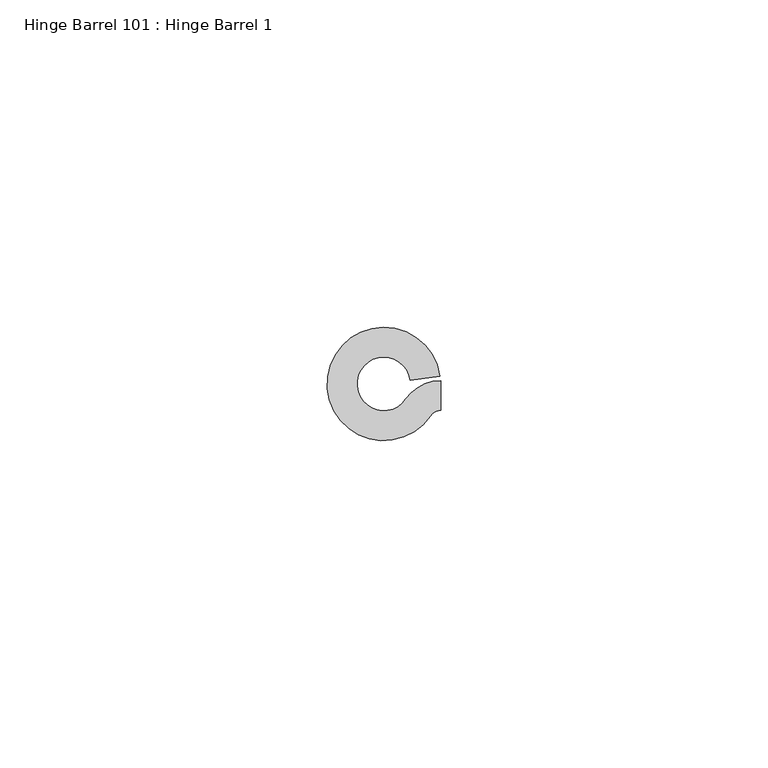
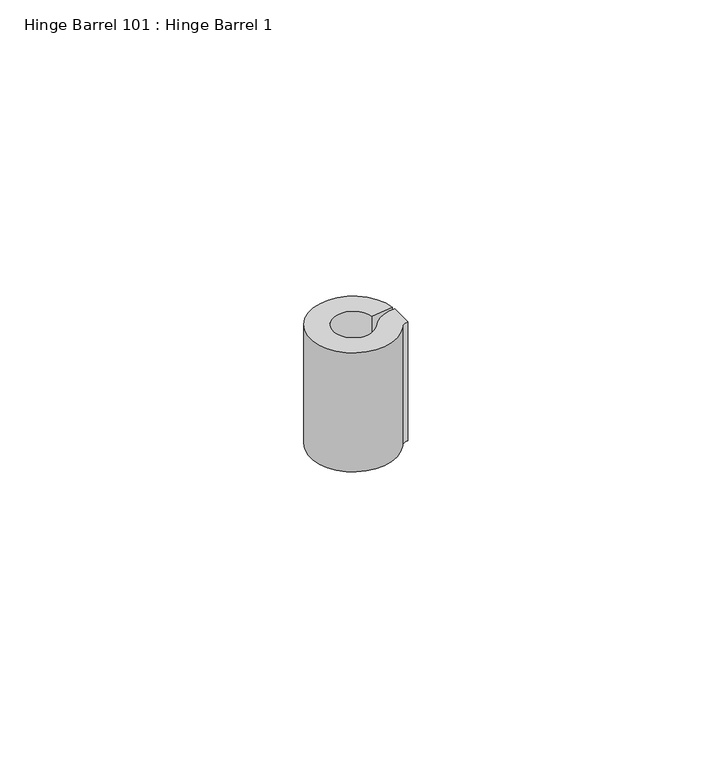
"""IFC4 building model written with IfcOpenShell, lengths in millimetres: proxy geometry, Hinge Barrel 101 : Hinge Barrel 1."""

import ifcopenshell
import ifcopenshell.guid

model = None  # the IFC model being written
_history = None  # IfcOwnerHistory: only IFC2X3 demands one
_inside = {}  # id of a spatial element -> (the spatial element, [elements in it])
_under = {}  # id of a project, library or spatial element -> (it, [spatial elements below it])
_declared = {}  # id of a project -> (the project, [libraries it declares])
_typed = {}  # id of a type object -> (the type object, [elements of that type])
_made_of = {}  # id of a material, layer set ... -> (it, [elements and type objects made of it])


def new_model(schema):
    """Start an empty IFC model of exactly this schema.

    Asked for "IFC4X3", IfcOpenShell would pick the latest addendum, in which some entities
    have other attributes; the version numbers below select the first issue.
    IFC2X3 requires an IfcOwnerHistory on every rooted entity: one is made here for all.
    """
    global model, _history
    if schema == "IFC4X3":
        model = ifcopenshell.file(schema_version=(4, 3, 0, 0))
    else:
        model = ifcopenshell.file(schema=schema)
    _inside.clear()
    _under.clear()
    _declared.clear()
    _typed.clear()
    _made_of.clear()
    _history = None
    if model.schema == "IFC2X3":
        org = make("IfcOrganization", Name="unknown")
        user = make(
            "IfcPersonAndOrganization",
            ThePerson=make("IfcPerson", FamilyName="unknown"),
            TheOrganization=org,
        )
        app = make(
            "IfcApplication",
            ApplicationDeveloper=org,
            Version="unknown",
            ApplicationFullName="unknown",
            ApplicationIdentifier="unknown",
        )
        _history = make(
            "IfcOwnerHistory",
            OwningUser=user,
            OwningApplication=app,
            ChangeAction="ADDED",
            CreationDate=0,
        )
    return model


def make(cls, **values):
    """One entity of the class cls with the attributes given. An attribute that is None is left unset."""
    return model.create_entity(
        cls, **{name: value for name, value in values.items() if value is not None}
    )


def rooted(cls, **values):
    """An entity with a GlobalId (a new one), such as an element, a storey or a relation."""
    return make(cls, GlobalId=ifcopenshell.guid.new(), OwnerHistory=_history, **values)


def si_unit(unit_type, name, prefix=None):
    """IfcSIUnit, for example si_unit("LENGTHUNIT", "METRE", prefix="MILLI")."""
    return make("IfcSIUnit", UnitType=unit_type, Prefix=prefix, Name=name)


def assignment(units):
    """IfcUnitAssignment: the units of a project."""
    return None if units is None else make("IfcUnitAssignment", Units=units)


def point(xyz):
    """IfcCartesianPoint."""
    return None if xyz is None else make("IfcCartesianPoint", Coordinates=xyz)


def direction(xyz):
    """IfcDirection."""
    return None if xyz is None else make("IfcDirection", DirectionRatios=xyz)


def frame(location, z_axis=None, x_axis=None):
    """IfcAxis2Placement3D, a coordinate frame: its origin and axes. An axis left out is left unset."""
    return make(
        "IfcAxis2Placement3D",
        Location=point(location),
        Axis=direction(z_axis),
        RefDirection=direction(x_axis),
    )


def frame_2d(location, x_axis=None):
    """IfcAxis2Placement2D, a coordinate frame in the plane: its origin and x axis."""
    return make(
        "IfcAxis2Placement2D", Location=point(location), RefDirection=direction(x_axis)
    )


def origin():
    """The frame at (0, 0, 0) with its axes left unset."""
    return frame((0.0, 0.0, 0.0))


def place(relative_to, where):
    """IfcLocalPlacement: puts the frame where relative to a parent placement (None: the world)."""
    return make(
        "IfcLocalPlacement", PlacementRelTo=relative_to, RelativePlacement=where
    )


def context(
    kind, dimensions, precision=None, world=None, true_north=None, identifier=None
):
    """IfcGeometricRepresentationContext, for example the 3D "Model" context."""
    return make(
        "IfcGeometricRepresentationContext",
        ContextIdentifier=identifier,
        ContextType=kind,
        CoordinateSpaceDimension=dimensions,
        Precision=precision,
        WorldCoordinateSystem=world,
        TrueNorth=true_north,
    )


def project(units=None, contexts=None):
    """IfcProject with its units and contexts."""
    return rooted(
        "IfcProject",
        Name="project",
        RepresentationContexts=contexts,
        UnitsInContext=assignment(units),
    )


def spatial(cls, under=None, at=None, **own):
    """A site, building, storey or space (cls), placed at a placement, below another one or the project."""
    s = rooted(cls, ObjectPlacement=at, **own)
    if under is not None:
        _under.setdefault(under.id(), (under, []))[1].append(s)
    return s


def polyline(points):
    """IfcPolyline through the points."""
    return make("IfcPolyline", Points=[point(p) for p in points])


def circle_curve(where, radius):
    """IfcCircle in the frame where."""
    return make("IfcCircle", Position=where, Radius=radius)


def trimmed(basis, trim1, trim2, sense, master):
    """IfcTrimmedCurve: the piece of a basis curve between two trims."""
    return make(
        "IfcTrimmedCurve",
        BasisCurve=basis,
        Trim1=trim1,
        Trim2=trim2,
        SenseAgreement=sense,
        MasterRepresentation=master,
    )


def segment(curve, same_sense, transition):
    """IfcCompositeCurveSegment."""
    return make(
        "IfcCompositeCurveSegment",
        Transition=transition,
        SameSense=same_sense,
        ParentCurve=curve,
    )


def composite_curve(segments, self_intersect=None):
    """IfcCompositeCurve: segments joined end to end."""
    return make("IfcCompositeCurve", Segments=segments, SelfIntersect=self_intersect)


def outline(outer, holes=None, kind="AREA"):
    """IfcArbitraryClosedProfileDef: a profile drawn as a closed curve; with holes, ...WithVoids."""
    if holes is None:
        return make("IfcArbitraryClosedProfileDef", ProfileType=kind, OuterCurve=outer)
    return make(
        "IfcArbitraryProfileDefWithVoids",
        ProfileType=kind,
        OuterCurve=outer,
        InnerCurves=holes,
    )


def extrude(swept, where, along, depth):
    """IfcExtrudedAreaSolid: the profile swept, set in the frame where, extruded along a direction by depth."""
    return make(
        "IfcExtrudedAreaSolid",
        SweptArea=swept,
        Position=where,
        ExtrudedDirection=direction(along),
        Depth=depth,
    )


def shape(context_of_items, identifier, shape_type, items):
    """IfcShapeRepresentation: the items that make up one representation, for example the "Body"."""
    return make(
        "IfcShapeRepresentation",
        ContextOfItems=context_of_items,
        RepresentationIdentifier=identifier,
        RepresentationType=shape_type,
        Items=items,
    )


def source(mapping_origin, context_of_items, identifier, shape_type, items):
    """IfcRepresentationMap: a shape defined once, which mapped items show again and again."""
    return make(
        "IfcRepresentationMap",
        MappingOrigin=mapping_origin,
        MappedRepresentation=shape(context_of_items, identifier, shape_type, items),
    )


def transform(
    local_origin,
    x_axis=None,
    y_axis=None,
    z_axis=None,
    scale=None,
    scale2=None,
    scale3=None,
    uniform=True,
):
    """IfcCartesianTransformationOperator3D, or its non-uniform kind. x_axis, y_axis, z_axis: its Axis1, 2, 3."""
    if uniform:
        return make(
            "IfcCartesianTransformationOperator3D",
            Axis1=direction(x_axis),
            Axis2=direction(y_axis),
            LocalOrigin=point(local_origin),
            Scale=scale,
            Axis3=direction(z_axis),
        )
    return make(
        "IfcCartesianTransformationOperator3DnonUniform",
        Axis1=direction(x_axis),
        Axis2=direction(y_axis),
        LocalOrigin=point(local_origin),
        Scale=scale,
        Axis3=direction(z_axis),
        Scale2=scale2,
        Scale3=scale3,
    )


def mapped(mapping_source, mapping_target):
    """IfcMappedItem: shows the shape of a source again, moved by a transform."""
    return make(
        "IfcMappedItem", MappingSource=mapping_source, MappingTarget=mapping_target
    )


def made_of(thing, what):
    """Note that an element or type object is made of a material, layer set ...; save() writes the relation."""
    if what is not None:
        _made_of.setdefault(what.id(), (what, []))[1].append(thing)
    return thing


def element(
    cls,
    number,
    at=None,
    inside=None,
    cuts=None,
    type_object=None,
    material=None,
    context=None,
    identifier="Body",
    shape_type=None,
    held_by="IfcProductDefinitionShape",
    body=None,
    shapes=None,
    **own,
):
    """One element of the class cls, such as IfcWall. Its Tag is "e" and its number.

    at: its placement. inside: the storey or other place that contains it. cuts: it is an
    opening in that element (IfcRelVoidsElement). A single representation is given by context,
    identifier, shape_type and body (its items); several are given by shapes. held_by: the class
    of the entity that holds the representations. save() writes the other relations.
    """
    e = rooted(cls, Tag="e%d" % number, ObjectPlacement=at, **own)
    if body is not None:
        shapes = [shape(context, identifier, shape_type, body)]
    if shapes is not None:
        e.Representation = make(held_by, Representations=shapes)
    if inside is not None:
        _inside.setdefault(inside.id(), (inside, []))[1].append(e)
    if cuts is not None:
        rooted(
            "IfcRelVoidsElement", RelatingBuildingElement=cuts, RelatedOpeningElement=e
        )
    if type_object is not None:
        _typed.setdefault(type_object.id(), (type_object, []))[1].append(e)
    return made_of(e, material)


def aggregate(whole, parts):
    """IfcRelAggregates: a whole, such as a stair, and the parts it consists of."""
    return rooted("IfcRelAggregates", RelatingObject=whole, RelatedObjects=parts)


def save(model, path):
    """Write the relations noted so far, then the file.

    IfcRelAggregates (storeys below a building ...), IfcRelContainedInSpatialStructure (elements
    in a storey), IfcRelDefinesByType, IfcRelAssociatesMaterial and IfcRelDeclares: one each for
    every whole, place, type object, material and project.
    """
    for whole, parts in _under.values():
        aggregate(whole, parts)
    for where, things in _inside.values():
        rooted(
            "IfcRelContainedInSpatialStructure",
            RelatedElements=things,
            RelatingStructure=where,
        )
    for kind, things in _typed.values():
        rooted("IfcRelDefinesByType", RelatedObjects=things, RelatingType=kind)
    for what, things in _made_of.values():
        rooted("IfcRelAssociatesMaterial", RelatedObjects=things, RelatingMaterial=what)
    for by, libraries in _declared.values():
        rooted("IfcRelDeclares", RelatingContext=by, RelatedDefinitions=libraries)
    model.write(path)


def hinge_barrel_101_hinge_barrel_1_6108b341(model_context):
    return source(origin(), model_context, "Body", "SweptSolid", [
        extrude(outline(composite_curve([segment(trimmed(circle_curve(frame_2d((587327.8245257, -533990.5568067)), 6.4044851), [point((587322.5194669, -533986.9688017))], [point((587327.8245257, -533984.1523216))], False, "CARTESIAN"), True, "CONTINUOUS"), segment(polyline([(587327.8245257, -533984.1523216), (587327.8245257, -533988.7163841)]), True, "CONTINUOUS"), segment(trimmed(circle_curve(frame_2d((587327.8245257, -533990.5568067)), 1.8404226), [point((587327.8245257, -533988.7163841))], [point((587326.3000393, -533989.5257409))], True, "CARTESIAN"), True, "CONTINUOUS"), segment(trimmed(circle_curve(frame_2d((587319.1320739, -533984.6777841)), 8.6534625), [point((587326.3000393, -533989.5257409))], [point((587327.7022899, -533983.4803654))], False, "CARTESIAN"), True, "CONTINUOUS"), segment(polyline([(587327.7022899, -533983.4803654), (587323.1821338, -533984.1119153)]), True, "CONTINUOUS"), segment(trimmed(circle_curve(frame_2d((587319.1320739, -533984.6777841)), 4.0894), [point((587323.1821338, -533984.1119153))], [point((587322.5194669, -533986.9688017))], True, "CARTESIAN"), True, "CONTINUOUS")], self_intersect=False)), frame((0.0, 0.0, 1962.15), z_axis=(0.0, 0.0, 1.0), x_axis=(1.0, 0.0, 0.0)), (0.0, 0.0, 1.0), 25.4),
    ])


if __name__ == "__main__":
    model = new_model("IFC4")
    model_context = context("Model", 3, world=origin())
    ifc_project = project(units=[si_unit("LENGTHUNIT", "METRE", prefix="MILLI")], contexts=[model_context])
    site = spatial("IfcSite", under=ifc_project)
    building = spatial("IfcBuilding", under=site)
    placement = place(None, origin())
    hinge_barrel_101_hinge_barrel_1_shape = hinge_barrel_101_hinge_barrel_1_6108b341(model_context)
    element("IfcBuildingElementProxy", 1, Name="Hinge Barrel 101 : Hinge Barrel 1", ObjectType="Hinge Barrel 101 : Hinge Barrel 1", at=placement, inside=building, context=model_context, shape_type="MappedRepresentation", body=[
        mapped(hinge_barrel_101_hinge_barrel_1_shape, transform((0.0, 0.0, 0.0), x_axis=(1.0, 0.0, 0.0), y_axis=(0.0, 1.0, 0.0), z_axis=(0.0, 0.0, 1.0))),
    ])
    save(model, "model.ifc")

# Revit data of these elements
# Element 1 (IfcBuildingElementProxy, "Hinge Barrel 101 : Hinge Barrel 1")
#   Materials on its faces: "6\"X6\" WELD-ON STL BUTT HINGE"
# Materials
#   "6\"X6\" WELD-ON STL BUTT HINGE": class "Metal", colour RGB 189 187 185, transparency 0, Description = "Carbon steel", Cost = 0
